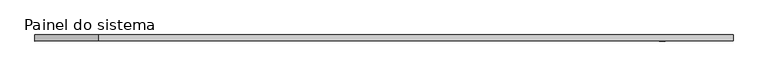
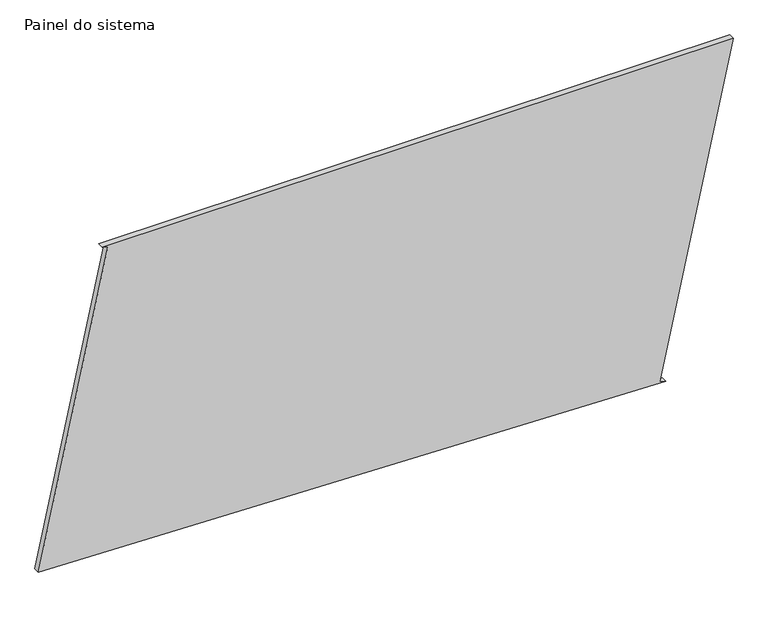
"""IFC4 building model written with IfcOpenShell, lengths in millimetres: plate geometry, Painel do sistema : Envidraçado."""

from ifc_helpers import new_model, si_unit, frame, origin, place, context, project, spatial, polyline, outline, extrude, source, transform, mapped, element, save


def painel_do_sistema_c6387456(model_context):
    return source(origin(), model_context, "Body", "SweptSolid", [
        extrude(outline(polyline([(0.0, 1156.4812402), (5.3087357, 1132.0513953), (1399.3021631, 1434.9736046), (1399.3021631, -1172.1130759), (1393.9934274, -1147.6832309), (71.9348913, -1434.9736046), (0.0, 1156.4812402)])), frame((0.0, 24.5, 0.0), z_axis=(0.0, 1.0, 0.0), x_axis=(0.0, 0.0, 1.0)), (0.0, 0.0, 1.0), 25.0),
    ])


if __name__ == "__main__":
    model = new_model("IFC4")
    model_context = context("Model", 3, world=origin())
    ifc_project = project(units=[si_unit("LENGTHUNIT", "METRE", prefix="MILLI")], contexts=[model_context])
    site = spatial("IfcSite", under=ifc_project)
    building = spatial("IfcBuilding", under=site)
    placement = place(None, origin())
    painel_do_sistema_shape = painel_do_sistema_c6387456(model_context)
    element("IfcPlate", 1, ObjectType="Painel do sistema : Envidraçado", at=placement, inside=building, context=model_context, shape_type="MappedRepresentation", body=[
        mapped(painel_do_sistema_shape, transform((0.0, 0.0, 0.0), x_axis=(1.0, 0.0, 0.0), y_axis=(0.0, 1.0, 0.0), z_axis=(0.0, 0.0, 1.0))),
    ])
    save(model, "model.ifc")

# Revit data of these elements
# Type "Painel do sistema : Envidraçado"
#   Construction Type Id = "GSP4R"
#   Analytic Construction = "Vidraça única Pilkington 1/8 pol"
#   Visual Light Transmittance = 0.9
#   Solar Heat Gain Coefficient = 0.86
#   Heat Transfer Coefficient (U) = 6.7069 W/(m²·K)
# Element 1 (IfcPlate, "Painel do sistema : Envidraçado")
#   Materials on its faces: "Vidro"
# Materials
#   "Vidro": class "Vidro", colour RGB 0 128 192, transparency 0.9, Description = "Vidro de sílica", Cost = 0
